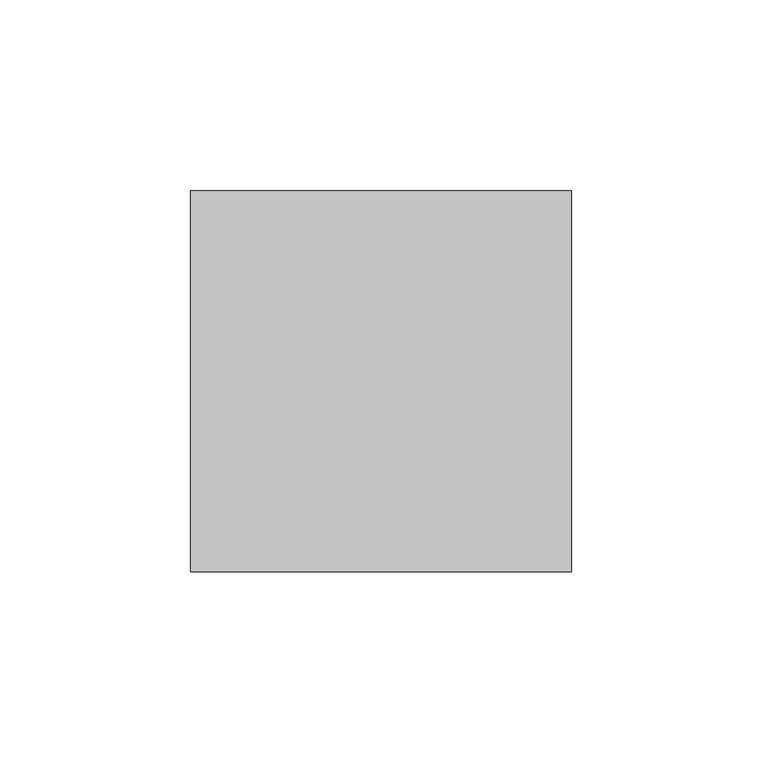
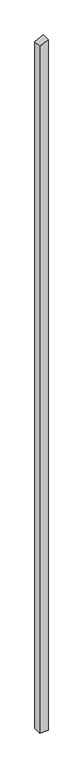
"""IFC4 building model written with IfcOpenShell, lengths in millimetres: column geometry, Holzstütze 158656 : Holzstütze 158656."""

from ifc_helpers import new_model, si_unit, frame, origin, place, context, project, spatial, polyline, outline, extrude, source, transform, mapped, element, save


def column_4b14859e(model_context):
    return source(origin(), model_context, "Body", "SweptSolid", [
        extrude(outline(polyline([(-500.0, 161027.7593015), (-500.0, 161127.7593015), (8297.1942973, 161127.7593015), (8246.2417524, 161027.7593015), (-500.0, 161027.7593015)])), frame((0.0, 47884.7962965, 0.0), z_axis=(0.0, 1.0, 0.0), x_axis=(0.0, 0.0, 1.0)), (0.0, 0.0, 1.0), 100.0),
    ])


if __name__ == "__main__":
    model = new_model("IFC4")
    model_context = context("Model", 3, world=origin())
    ifc_project = project(units=[si_unit("LENGTHUNIT", "METRE", prefix="MILLI")], contexts=[model_context])
    site = spatial("IfcSite", under=ifc_project)
    building = spatial("IfcBuilding", under=site)
    placement = place(None, origin())
    column_shape = column_4b14859e(model_context)
    element("IfcColumn", 1, ObjectType="Holzstütze 158656 : Holzstütze 158656", at=placement, inside=building, context=model_context, shape_type="MappedRepresentation", body=[
        mapped(column_shape, transform((0.0, 0.0, 0.0), x_axis=(1.0, 0.0, 0.0), y_axis=(0.0, 1.0, 0.0), z_axis=(0.0, 0.0, 1.0))),
    ])
    save(model, "model.ifc")

# Revit data of these elements
# Type "Holzstütze 158656 : Holzstütze 158656"
#   Abrechnungsart = "m"
#   Allright_Bauteil_ID = "0152St 0000143543"
#   Bezeichnung = "Holzstütze"
#   Codetext = "ST-HOLZ\\"
#   Gewerk = "Zimmer- und Holzbauarbeiten"
#   Material = "Holz"
#   Objektname = "Stütze"
#   NameOverride = "Holzstütze"
#   Reference = "Holzstütze"
#   Status = "NEW"
#   ThermalTransmittance = 0.0000 BTU/(h·ft²·°F)
#   Roll = 0.00°
#   Slope = 0.00°
#   2D Interaktion = yes
#   IsExternal = yes
#   LoadBearing = yes
# Element 1 (IfcColumn, "Holzstütze 158656 : Holzstütze 158656")
#   Materials on its faces: "holzschalung"
# Materials
#   "holzschalung": class "Unassigned", colour RGB 128 128 128, transparency 0
